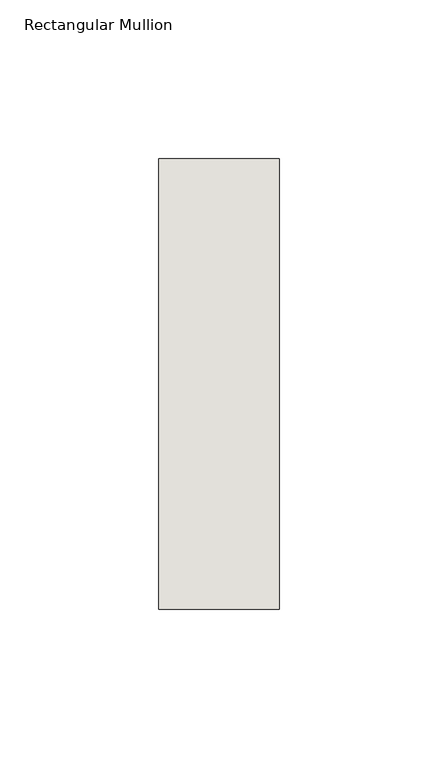
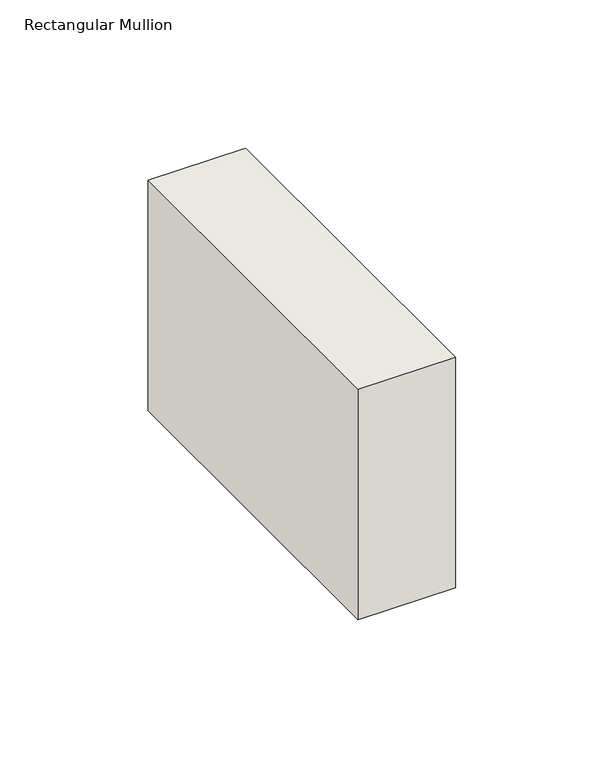
"""IFC4 building model written with IfcOpenShell, lengths in millimetres: wall geometry, Rectangular Mullion : NLRS_21_CWM_hsb-regel 38x142_gen_rsf."""

from ifc_helpers import new_model, si_unit, frame, origin, place, context, project, spatial, polyline, outline, extrude, source, transform, mapped, element, save


def rectangular_mullion_d3b03aeb(model_context):
    return source(origin(), model_context, "Body", "SweptSolid", [
        extrude(outline(polyline([(0.0, -71.0), (-38.0, -71.0), (-38.0, 71.0), (0.0, 71.0), (0.0, -71.0)])), frame((0.0, 0.0, -94.9999997), z_axis=(0.0, 0.0, 1.0), x_axis=(1.0, 0.0, 0.0)), (0.0, 0.0, 1.0), 94.9999997),
    ])


if __name__ == "__main__":
    model = new_model("IFC4")
    model_context = context("Model", 3, world=origin())
    ifc_project = project(units=[si_unit("LENGTHUNIT", "METRE", prefix="MILLI")], contexts=[model_context])
    site = spatial("IfcSite", under=ifc_project)
    building = spatial("IfcBuilding", under=site)
    placement = place(None, origin())
    rectangular_mullion_shape = rectangular_mullion_d3b03aeb(model_context)
    element("IfcWall", 1, ObjectType="Rectangular Mullion : NLRS_21_CWM_hsb-regel 38x142_gen_rsf", at=placement, inside=building, context=model_context, shape_type="MappedRepresentation", body=[
        mapped(rectangular_mullion_shape, transform((0.0, 0.0, 0.0), x_axis=(1.0, 0.0, 0.0), y_axis=(0.0, 1.0, 0.0), z_axis=(0.0, 0.0, 1.0))),
    ])
    save(model, "model.ifc")

# Revit data of these elements
# Type "Rectangular Mullion : NLRS_21_CWM_hsb-regel 38x142_gen_rsf"
#   Type IfcGUID = "07M7mRoiH1CR8m_RSKIwpF"
#   Assembly Code = "21.10"
#   IfcExportAs = "IfcWall"
#   built-in parameter 1007322 = 0.465879 (stored number, unit not read)
#   built-in parameter 1007321 = 0.062336 (stored number, unit not read)
#   built-in parameter 1007320 = 0.062336 (stored number, unit not read)
# Element 1 (IfcWall, "Rectangular Mullion : NLRS_21_CWM_hsb-regel 38x142_gen_rsf")
#   Materials on its faces: "NLRS_i2_hout naaldhout vuren_gen_rsf"
# Materials
#   "NLRS_i2_hout naaldhout vuren_gen_rsf": class "I - Hout", colour RGB 234 199 147, transparency 0, Keynote = "i2", Manufacturer = "Revit Standards Foundation", URL = "www.revitstandards.org", Description = "hout vuren", Cost = 0
